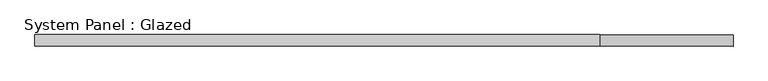
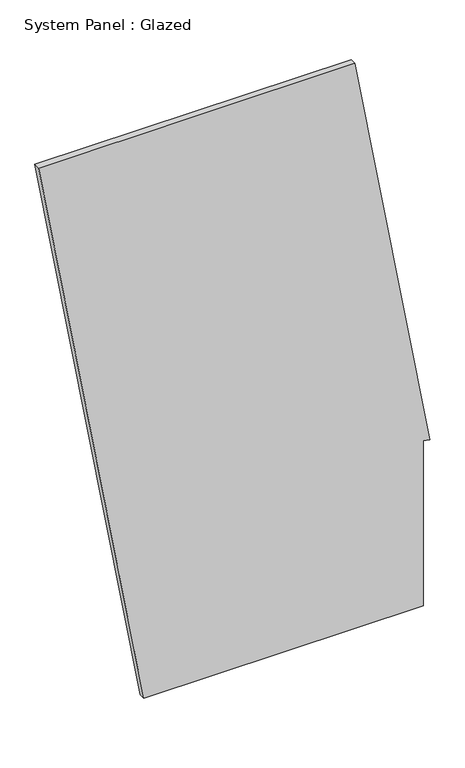
"""IFC4 building model written with IfcOpenShell, lengths in millimetres: plate geometry, System Panel : Glazed."""

from ifc_helpers import new_model, si_unit, frame, origin, place, context, project, spatial, polyline, outline, extrude, source, transform, mapped, element, save


def system_panel_glazed_902a334c(model_context):
    return source(origin(), model_context, "Body", "SweptSolid", [
        extrude(outline(polyline([(0.0, -351.2403762), (0.0, 735.8208002), (678.7181793, 735.8208002), (674.3769749, 761.2006064), (2325.0, 470.1512321), (2325.0, -761.2006064), (0.0, -351.2403762)])), frame((0.0, -49.5, 0.0), z_axis=(0.0, 1.0, 0.0), x_axis=(0.0, 0.0, 1.0)), (0.0, 0.0, 1.0), 25.0),
    ])


if __name__ == "__main__":
    model = new_model("IFC4")
    model_context = context("Model", 3, world=origin())
    ifc_project = project(units=[si_unit("LENGTHUNIT", "METRE", prefix="MILLI")], contexts=[model_context])
    site = spatial("IfcSite", under=ifc_project)
    building = spatial("IfcBuilding", under=site)
    placement = place(None, origin())
    system_panel_glazed_shape = system_panel_glazed_902a334c(model_context)
    element("IfcPlate", 1, ObjectType="System Panel : Glazed", at=placement, inside=building, context=model_context, shape_type="MappedRepresentation", body=[
        mapped(system_panel_glazed_shape, transform((0.0, 0.0, 0.0), x_axis=(1.0, 0.0, 0.0), y_axis=(0.0, 1.0, 0.0), z_axis=(0.0, 0.0, 1.0))),
    ])
    save(model, "model.ifc")

# Revit data of these elements
# Type "System Panel : Glazed"
#   Construction Type Id = "GSP4R"
#   Analytic Construction = "1/8 in Pilkington single glazing"
#   Visual Light Transmittance = 0.9
#   Solar Heat Gain Coefficient = 0.86
#   Heat Transfer Coefficient (U) = 6.7069 W/(m²·K)
#   Define Thermal Properties by = 1
# Element 1 (IfcPlate, "System Panel : Glazed")
#   Materials on its faces: "Glass"
# Materials
#   "Glass": class "Glass", colour RGB 0 128 192, transparency 0.9, Description = "Soda Lime Glass", Cost = 0
